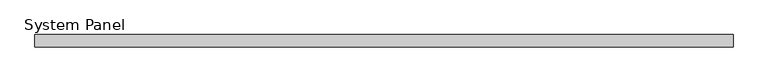
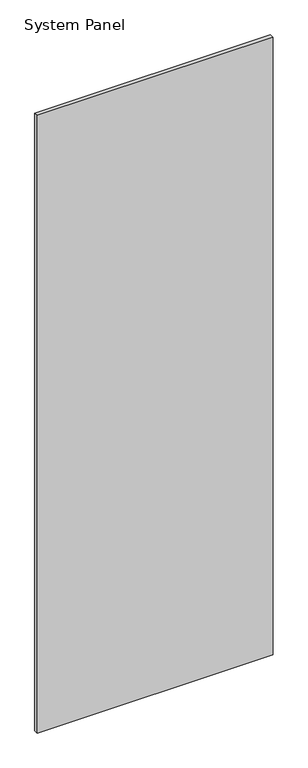
"""IFC4 building model written with IfcOpenShell, lengths in millimetres: plate geometry, System Panel : WWm-Glass-20mm-10mmOffset."""

from ifc_helpers import new_model, si_unit, origin, origin_with_axes, place, context, project, spatial, polyline, outline, extrude, source, transform, mapped, element, save


def system_panel_f8841630(model_context):
    return source(origin(), model_context, "Body", "SweptSolid", [
        extrude(outline(polyline([(569.3846306, 0.0), (-569.3846306, 0.0), (-569.3846306, 20.0), (569.3846306, 20.0), (569.3846306, 0.0)])), origin_with_axes(), (0.0, 0.0, 1.0), 3150.0),
    ])


if __name__ == "__main__":
    model = new_model("IFC4")
    model_context = context("Model", 3, world=origin())
    ifc_project = project(units=[si_unit("LENGTHUNIT", "METRE", prefix="MILLI")], contexts=[model_context])
    site = spatial("IfcSite", under=ifc_project)
    building = spatial("IfcBuilding", under=site)
    placement = place(None, origin())
    system_panel_shape = system_panel_f8841630(model_context)
    element("IfcPlate", 1, ObjectType="System Panel : WWm-Glass-20mm-10mmOffset", at=placement, inside=building, context=model_context, shape_type="MappedRepresentation", body=[
        mapped(system_panel_shape, transform((0.0, 0.0, 0.0), x_axis=(1.0, 0.0, 0.0), y_axis=(0.0, 1.0, 0.0), z_axis=(0.0, 0.0, 1.0))),
    ])
    save(model, "model.ifc")

# Revit data of these elements
# Type "System Panel : WWm-Glass-20mm-10mmOffset"
#   Finish = ""
# Element 1 (IfcPlate, "System Panel : WWm-Glass-20mm-10mmOffset")
#   Materials on its faces: "WW-EC-GL-Storefront"
# Materials
#   "WW-EC-GL-Storefront": class "Glass", colour RGB 236 240 239, transparency 0.85, Description = "Storefront Glass", Cost = 0
